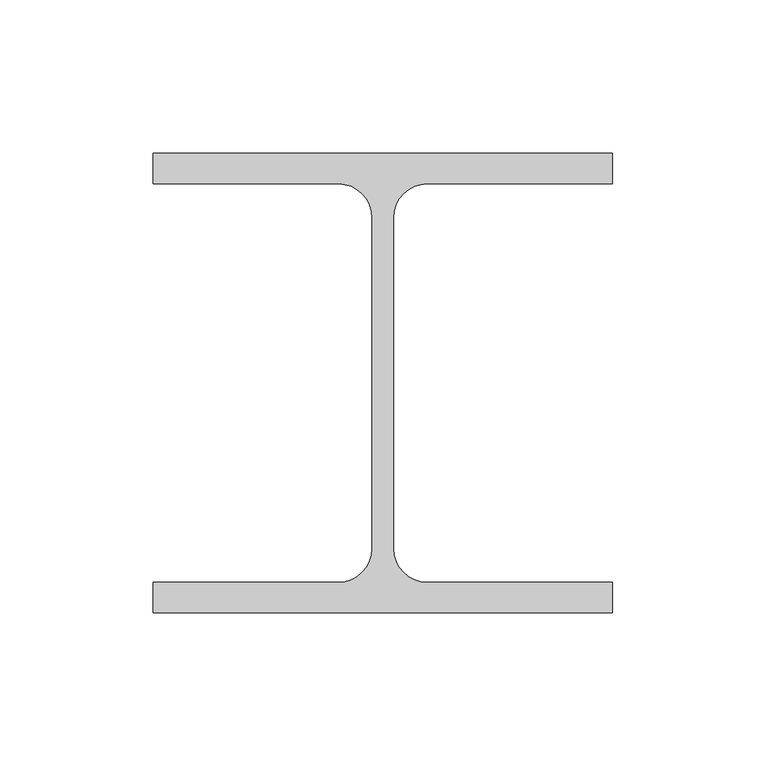
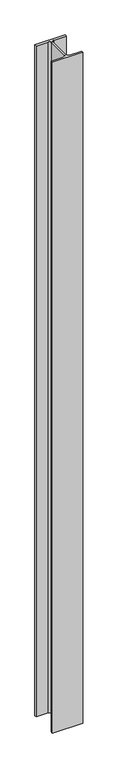
"""IFC4 building model written with IfcOpenShell, lengths in millimetres: column geometry, 0912_Steel Column_H_KSD3502 : H_SC_ASC_H-150x150x7x10."""

from ifc_helpers import new_model, si_unit, point, frame, frame_2d, origin, place, context, project, spatial, polyline, circle_curve, trimmed, segment, composite_curve, outline, extrude, source, transform, mapped, element, save


def column_e739ab66(model_context):
    return source(origin(), model_context, "Body", "SweptSolid", [
        extrude(outline(composite_curve([segment(polyline([(75.0, 75.0), (75.0, 65.0), (14.5, 65.0)]), True, "CONTINUOUS"), segment(trimmed(circle_curve(frame_2d((14.5, 54.0)), 11.0), [point((14.5, 65.0))], [point((3.5, 54.0))], True, "CARTESIAN"), True, "CONTINUOUS"), segment(polyline([(3.5, 54.0), (3.5, -54.0)]), True, "CONTINUOUS"), segment(trimmed(circle_curve(frame_2d((14.5, -54.0)), 11.0), [point((3.5, -54.0))], [point((14.5, -65.0))], True, "CARTESIAN"), True, "CONTINUOUS"), segment(polyline([(14.5, -65.0), (75.0, -65.0), (75.0, -75.0), (-75.0, -75.0), (-75.0, -65.0), (-14.5, -65.0)]), True, "CONTINUOUS"), segment(trimmed(circle_curve(frame_2d((-14.5, -54.0)), 11.0), [point((-14.5, -65.0))], [point((-3.5, -54.0))], True, "CARTESIAN"), True, "CONTINUOUS"), segment(polyline([(-3.5, -54.0), (-3.5, 54.0)]), True, "CONTINUOUS"), segment(trimmed(circle_curve(frame_2d((-14.5, 54.0)), 11.0), [point((-3.5, 54.0))], [point((-14.5, 65.0))], True, "CARTESIAN"), True, "CONTINUOUS"), segment(polyline([(-14.5, 65.0), (-75.0, 65.0), (-75.0, 75.0), (75.0, 75.0)]), True, "CONTINUOUS")], self_intersect=False)), frame((0.0, 0.0, 599.9720055), z_axis=(0.0, 0.0, 1.0), x_axis=(1.0, 0.0, 0.0)), (0.0, 0.0, 1.0), 3510.0),
    ])


if __name__ == "__main__":
    model = new_model("IFC4")
    model_context = context("Model", 3, world=origin())
    ifc_project = project(units=[si_unit("LENGTHUNIT", "METRE", prefix="MILLI")], contexts=[model_context])
    site = spatial("IfcSite", under=ifc_project)
    building = spatial("IfcBuilding", under=site)
    placement = place(None, origin())
    column_shape = column_e739ab66(model_context)
    element("IfcColumn", 1, ObjectType="0912_Steel Column_H_KSD3502 : H_SC_ASC_H-150x150x7x10", at=placement, inside=building, context=model_context, shape_type="MappedRepresentation", body=[
        mapped(column_shape, transform((0.0, 0.0, 0.0), x_axis=(1.0, 0.0, 0.0), y_axis=(0.0, 1.0, 0.0), z_axis=(0.0, 0.0, 1.0))),
    ])
    save(model, "model.ifc")

# Revit data of these elements
# Type "0912_Steel Column_H_KSD3502 : H_SC_ASC_H-150x150x7x10"
#   H_WM Code_1 = "S01AA002-00001 | Main Steel Structure Fabrication Work | Shelter/Building | Medium Steel - Standard (90KG/M>Weight≥30KG/M) | Material: (   )"
#   H_WM Code_2 = "S03AA028-00001 | Main Steel Structure Erection Work | Shelter/Building | Medium Steel (90KG/M>Weight≥30KG/M) | Material: (   )"
#   H_WM Code_3 = "S01AA010-00001 | Main Steel Structure Fabrication Work | Shelter/Building | Steel Painting/Coating | for Non-Fireproofed Steel Surface, Surface Preparation, Primer, Second & Final Coat | Material: (   )"
#   H_Q'ty Cal Type Tag = "SC-Q2"
#   Width = 15.0 cm
#   Web Thickness = 0.7 cm
#   Web Fillet = 1.1 cm
#   Warping Constant = 27562.5 cm⁶
#   Torsional Moment of Inertia = 11.6007 cm⁴
#   Section Area = 40.14 cm²
#   Plastic Modulus weak axis = 115.0 cm³
#   Plastic Modulus strong axis = 246.0 cm³
#   Perimeter = 0.87 m²/m
#   Nominal Weight = 31.50 kgf/m
#   Moment of Inertia weak axis = 563.00 cm⁴
#   Moment of Inertia strong axis = 1640.00 cm⁴
#   Height = 15.0 cm
#   Flange Thickness = 1.0 cm
#   Elastic Modulus weak axis = 75.1 cm³
#   Elastic Modulus strong axis = 219.0 cm³
#   Centroid Vertical = 7.5 cm
#   Centroid Horizontal = 7.5 cm
#   Structural Material [instance default] = Steel, 45-345
#   Section Name Key = ""
#   Bolt Spacing = 0
#   Assembly Code = ""
# Element 1 (IfcColumn, "0912_Steel Column_H_KSD3502 : H_SC_ASC_H-150x150x7x10")
#   Structural Material = A03AD029-00005_Anchor Bolt (Installation only)_M24
#   Materials on its faces: "A03AD029-00005_Anchor Bolt (Installation only)_M24"
# Materials
#   "Steel, 45-345": class "Metal", colour RGB 189 187 185, transparency 0, Description = "Steel 345 MPa", Cost = 0
#   "A03AD029-00005_Anchor Bolt (Installation only)_M24": class "Unassigned", colour RGB 84 83 81, transparency 0, Cost = 0
